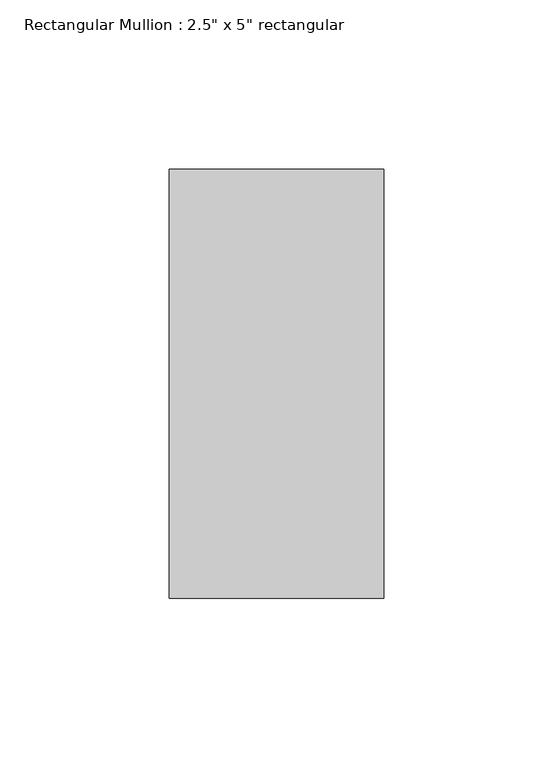
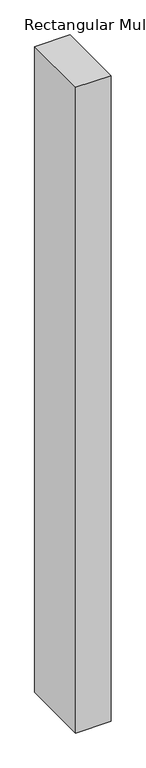
"""IFC4 building model written with IfcOpenShell, lengths in millimetres: member geometry."""

from ifc_helpers import new_model, si_unit, frame, origin, place, context, project, spatial, polyline, outline, extrude, source, transform, mapped, element, save


def member_9aff912a(model_context):
    return source(origin(), model_context, "Body", "SweptSolid", [
        extrude(outline(polyline([(31.75, 63.5), (31.75, -63.5), (-31.75, -63.5), (-31.75, 63.5), (31.75, 63.5)])), frame((0.0, 0.0, -1220.5651287), z_axis=(0.0, 0.0, 1.0), x_axis=(1.0, 0.0, 0.0)), (0.0, 0.0, 1.0), 1220.5651287),
    ])


if __name__ == "__main__":
    model = new_model("IFC4")
    model_context = context("Model", 3, world=origin())
    ifc_project = project(units=[si_unit("LENGTHUNIT", "METRE", prefix="MILLI")], contexts=[model_context])
    site = spatial("IfcSite", under=ifc_project)
    building = spatial("IfcBuilding", under=site)
    placement = place(None, origin())
    member_shape = member_9aff912a(model_context)
    element("IfcMember", 1, ObjectType="Rectangular Mullion : 2.5\" x 5\" rectangular", at=placement, inside=building, context=model_context, shape_type="MappedRepresentation", body=[
        mapped(member_shape, transform((0.0, 0.0, 0.0), x_axis=(1.0, 0.0, 0.0), y_axis=(0.0, 1.0, 0.0), z_axis=(0.0, 0.0, 1.0))),
    ])
    save(model, "model.ifc")

# Revit data of these elements
# Type "Rectangular Mullion : 2.5\" x 5\" rectangular"
#   built-in parameter 1007304 = 0.416667 (stored number, unit not read)
#   built-in parameter 1007301 = 0.104167 (stored number, unit not read)
#   built-in parameter 1007300 = 0.104167 (stored number, unit not read)
# Element 1 (IfcMember, "Rectangular Mullion : 2.5\" x 5\" rectangular")
#   Materials on its faces: "Metal - Aluminum"
# Materials
#   "Metal - Aluminum": class "Metal", colour RGB 140 140 140, transparency 0
